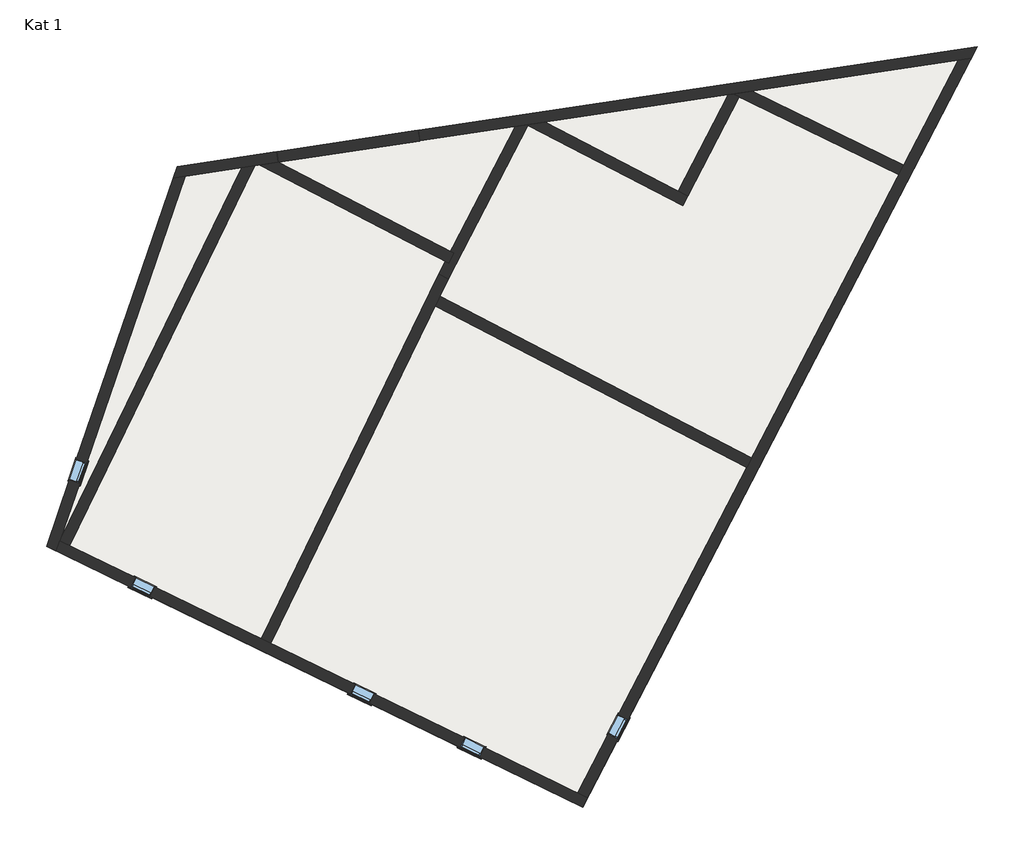
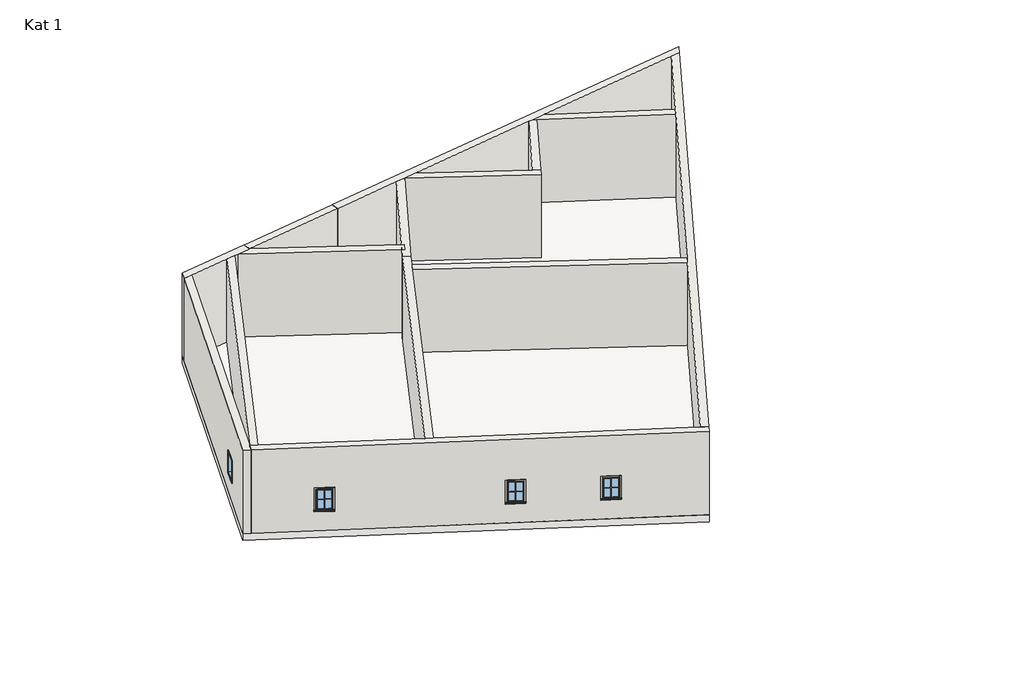
# One storey: 15 proxies, 14 walls, 5 windows, 1 slab.
"""IFC4 building model written with IfcOpenShell, lengths in millimetres."""

import ifcopenshell
import ifcopenshell.guid

model = None  # the IFC model being written
_history = None  # IfcOwnerHistory: only IFC2X3 demands one
_inside = {}  # id of a spatial element -> (the spatial element, [elements in it])
_under = {}  # id of a project, library or spatial element -> (it, [spatial elements below it])
_declared = {}  # id of a project -> (the project, [libraries it declares])
_typed = {}  # id of a type object -> (the type object, [elements of that type])
_made_of = {}  # id of a material, layer set ... -> (it, [elements and type objects made of it])


def new_model(schema):
    """Start an empty IFC model of exactly this schema.

    Asked for "IFC4X3", IfcOpenShell would pick the latest addendum, in which some entities
    have other attributes; the version numbers below select the first issue.
    IFC2X3 requires an IfcOwnerHistory on every rooted entity: one is made here for all.
    """
    global model, _history
    if schema == "IFC4X3":
        model = ifcopenshell.file(schema_version=(4, 3, 0, 0))
    else:
        model = ifcopenshell.file(schema=schema)
    _inside.clear()
    _under.clear()
    _declared.clear()
    _typed.clear()
    _made_of.clear()
    _history = None
    if model.schema == "IFC2X3":
        org = make("IfcOrganization", Name="unknown")
        user = make(
            "IfcPersonAndOrganization",
            ThePerson=make("IfcPerson", FamilyName="unknown"),
            TheOrganization=org,
        )
        app = make(
            "IfcApplication",
            ApplicationDeveloper=org,
            Version="unknown",
            ApplicationFullName="unknown",
            ApplicationIdentifier="unknown",
        )
        _history = make(
            "IfcOwnerHistory",
            OwningUser=user,
            OwningApplication=app,
            ChangeAction="ADDED",
            CreationDate=0,
        )
    return model


def make(cls, **values):
    """One entity of the class cls with the attributes given. An attribute that is None is left unset."""
    return model.create_entity(
        cls, **{name: value for name, value in values.items() if value is not None}
    )


def rooted(cls, **values):
    """An entity with a GlobalId (a new one), such as an element, a storey or a relation."""
    return make(cls, GlobalId=ifcopenshell.guid.new(), OwnerHistory=_history, **values)


def si_unit(unit_type, name, prefix=None):
    """IfcSIUnit, for example si_unit("LENGTHUNIT", "METRE", prefix="MILLI")."""
    return make("IfcSIUnit", UnitType=unit_type, Prefix=prefix, Name=name)


def assignment(units):
    """IfcUnitAssignment: the units of a project."""
    return None if units is None else make("IfcUnitAssignment", Units=units)


def point(xyz):
    """IfcCartesianPoint."""
    return None if xyz is None else make("IfcCartesianPoint", Coordinates=xyz)


def direction(xyz):
    """IfcDirection."""
    return None if xyz is None else make("IfcDirection", DirectionRatios=xyz)


def frame(location, z_axis=None, x_axis=None):
    """IfcAxis2Placement3D, a coordinate frame: its origin and axes. An axis left out is left unset."""
    return make(
        "IfcAxis2Placement3D",
        Location=point(location),
        Axis=direction(z_axis),
        RefDirection=direction(x_axis),
    )


def origin():
    """The frame at (0, 0, 0) with its axes left unset."""
    return frame((0.0, 0.0, 0.0))


def origin_with_axes():
    """The frame at (0, 0, 0) with the z axis (0, 0, 1) and the x axis (1, 0, 0) written out."""
    return frame((0.0, 0.0, 0.0), z_axis=(0.0, 0.0, 1.0), x_axis=(1.0, 0.0, 0.0))


def place(relative_to, where):
    """IfcLocalPlacement: puts the frame where relative to a parent placement (None: the world)."""
    return make(
        "IfcLocalPlacement", PlacementRelTo=relative_to, RelativePlacement=where
    )


def context(
    kind, dimensions, precision=None, world=None, true_north=None, identifier=None
):
    """IfcGeometricRepresentationContext, for example the 3D "Model" context."""
    return make(
        "IfcGeometricRepresentationContext",
        ContextIdentifier=identifier,
        ContextType=kind,
        CoordinateSpaceDimension=dimensions,
        Precision=precision,
        WorldCoordinateSystem=world,
        TrueNorth=true_north,
    )


def project(units=None, contexts=None):
    """IfcProject with its units and contexts."""
    return rooted(
        "IfcProject",
        Name="project",
        RepresentationContexts=contexts,
        UnitsInContext=assignment(units),
    )


def spatial(cls, under=None, at=None, **own):
    """A site, building, storey or space (cls), placed at a placement, below another one or the project."""
    s = rooted(cls, ObjectPlacement=at, **own)
    if under is not None:
        _under.setdefault(under.id(), (under, []))[1].append(s)
    return s


def polyline(points):
    """IfcPolyline through the points."""
    return make("IfcPolyline", Points=[point(p) for p in points])


def outline(outer, holes=None, kind="AREA"):
    """IfcArbitraryClosedProfileDef: a profile drawn as a closed curve; with holes, ...WithVoids."""
    if holes is None:
        return make("IfcArbitraryClosedProfileDef", ProfileType=kind, OuterCurve=outer)
    return make(
        "IfcArbitraryProfileDefWithVoids",
        ProfileType=kind,
        OuterCurve=outer,
        InnerCurves=holes,
    )


def extrude(swept, where, along, depth):
    """IfcExtrudedAreaSolid: the profile swept, set in the frame where, extruded along a direction by depth."""
    return make(
        "IfcExtrudedAreaSolid",
        SweptArea=swept,
        Position=where,
        ExtrudedDirection=direction(along),
        Depth=depth,
    )


def faces_of(points, faces, orient=None, outer=None):
    """IfcFace entities. A face is a list of loops; a loop is a list of indices into points, from 0.

    orient and outer hold one flag for each loop. By default every Orientation is true, the
    first loop of a face is its IfcFaceOuterBound and the others are IfcFaceBound.
    """
    made = []
    for i, loops in enumerate(faces):
        bounds = []
        for j, loop in enumerate(loops):
            is_outer = j == 0 if outer is None else outer[i][j]
            bounds.append(
                make(
                    "IfcFaceOuterBound" if is_outer else "IfcFaceBound",
                    Bound=make("IfcPolyLoop", Polygon=[points[k] for k in loop]),
                    Orientation=True if orient is None else orient[i][j],
                )
            )
        made.append(make("IfcFace", Bounds=bounds))
    return made


def faceted_brep(points, faces, orient=None, outer=None, voids=None):
    """IfcFacetedBrep: a solid bounded by flat faces; with voids (closed shells), ...WithVoids."""
    shared = [point(p) for p in points]
    hull = make("IfcClosedShell", CfsFaces=faces_of(shared, faces, orient, outer))
    if voids is None:
        return make("IfcFacetedBrep", Outer=hull)
    return make(
        "IfcFacetedBrepWithVoids",
        Outer=hull,
        Voids=[
            make(cls, CfsFaces=faces_of(shared, fs, o, b)) for cls, fs, o, b in voids
        ],
    )


def shape(context_of_items, identifier, shape_type, items):
    """IfcShapeRepresentation: the items that make up one representation, for example the "Body"."""
    return make(
        "IfcShapeRepresentation",
        ContextOfItems=context_of_items,
        RepresentationIdentifier=identifier,
        RepresentationType=shape_type,
        Items=items,
    )


def source(mapping_origin, context_of_items, identifier, shape_type, items):
    """IfcRepresentationMap: a shape defined once, which mapped items show again and again."""
    return make(
        "IfcRepresentationMap",
        MappingOrigin=mapping_origin,
        MappedRepresentation=shape(context_of_items, identifier, shape_type, items),
    )


def transform(
    local_origin,
    x_axis=None,
    y_axis=None,
    z_axis=None,
    scale=None,
    scale2=None,
    scale3=None,
    uniform=True,
):
    """IfcCartesianTransformationOperator3D, or its non-uniform kind. x_axis, y_axis, z_axis: its Axis1, 2, 3."""
    if uniform:
        return make(
            "IfcCartesianTransformationOperator3D",
            Axis1=direction(x_axis),
            Axis2=direction(y_axis),
            LocalOrigin=point(local_origin),
            Scale=scale,
            Axis3=direction(z_axis),
        )
    return make(
        "IfcCartesianTransformationOperator3DnonUniform",
        Axis1=direction(x_axis),
        Axis2=direction(y_axis),
        LocalOrigin=point(local_origin),
        Scale=scale,
        Axis3=direction(z_axis),
        Scale2=scale2,
        Scale3=scale3,
    )


def mapped(mapping_source, mapping_target):
    """IfcMappedItem: shows the shape of a source again, moved by a transform."""
    return make(
        "IfcMappedItem", MappingSource=mapping_source, MappingTarget=mapping_target
    )


def made_of(thing, what):
    """Note that an element or type object is made of a material, layer set ...; save() writes the relation."""
    if what is not None:
        _made_of.setdefault(what.id(), (what, []))[1].append(thing)
    return thing


def element(
    cls,
    number,
    at=None,
    inside=None,
    cuts=None,
    type_object=None,
    material=None,
    context=None,
    identifier="Body",
    shape_type=None,
    held_by="IfcProductDefinitionShape",
    body=None,
    shapes=None,
    **own,
):
    """One element of the class cls, such as IfcWall. Its Tag is "e" and its number.

    at: its placement. inside: the storey or other place that contains it. cuts: it is an
    opening in that element (IfcRelVoidsElement). A single representation is given by context,
    identifier, shape_type and body (its items); several are given by shapes. held_by: the class
    of the entity that holds the representations. save() writes the other relations.
    """
    e = rooted(cls, Tag="e%d" % number, ObjectPlacement=at, **own)
    if body is not None:
        shapes = [shape(context, identifier, shape_type, body)]
    if shapes is not None:
        e.Representation = make(held_by, Representations=shapes)
    if inside is not None:
        _inside.setdefault(inside.id(), (inside, []))[1].append(e)
    if cuts is not None:
        rooted(
            "IfcRelVoidsElement", RelatingBuildingElement=cuts, RelatedOpeningElement=e
        )
    if type_object is not None:
        _typed.setdefault(type_object.id(), (type_object, []))[1].append(e)
    return made_of(e, material)


def aggregate(whole, parts):
    """IfcRelAggregates: a whole, such as a stair, and the parts it consists of."""
    return rooted("IfcRelAggregates", RelatingObject=whole, RelatedObjects=parts)


def save(model, path):
    """Write the relations noted so far, then the file.

    IfcRelAggregates (storeys below a building ...), IfcRelContainedInSpatialStructure (elements
    in a storey), IfcRelDefinesByType, IfcRelAssociatesMaterial and IfcRelDeclares: one each for
    every whole, place, type object, material and project.
    """
    for whole, parts in _under.values():
        aggregate(whole, parts)
    for where, things in _inside.values():
        rooted(
            "IfcRelContainedInSpatialStructure",
            RelatedElements=things,
            RelatingStructure=where,
        )
    for kind, things in _typed.values():
        rooted("IfcRelDefinesByType", RelatedObjects=things, RelatingType=kind)
    for what, things in _made_of.values():
        rooted("IfcRelAssociatesMaterial", RelatedObjects=things, RelatingMaterial=what)
    for by, libraries in _declared.values():
        rooted("IfcRelDeclares", RelatingContext=by, RelatedDefinitions=libraries)
    model.write(path)


def m_muntin_pattern_2x2_m_muntin_pattern_2x2_8a7fc2d2(model_context):
    return source(origin(), model_context, "Body", "SweptSolid", [
        extrude(outline(polyline([(418.25, -6.35), (418.25, -261.9), (405.55, -261.9), (405.55, -6.35), (0.0, -6.35), (0.0, 6.35), (405.55, 6.35), (405.55, 261.9), (418.25, 261.9), (418.25, 6.35), (823.8, 6.35), (823.8, -6.35), (418.25, -6.35)])), frame((0.0, -22.225, 0.0), z_axis=(0.0, 1.0, 0.0), x_axis=(0.0, 0.0, 1.0)), (0.0, 0.0, 1.0), 12.7),
        extrude(outline(polyline([(418.25, -6.35), (418.25, -261.9), (405.55, -261.9), (405.55, -6.35), (0.0, -6.35), (0.0, 6.35), (405.55, 6.35), (405.55, 261.9), (418.25, 261.9), (418.25, 6.35), (823.8, 6.35), (823.8, -6.35), (418.25, -6.35)])), frame((0.0, 9.525, 0.0), z_axis=(0.0, 1.0, 0.0), x_axis=(0.0, 0.0, 1.0)), (0.0, 0.0, 1.0), 12.7),
    ])


def m_trim_window_exterior_flat_with_sill_a9fd4a74(model_context):
    return source(origin(), model_context, "Body", "SweptSolid", [
        extrude(outline(polyline([(360.0, -920.4323709), (360.0, -980.4323709), (-360.0, -980.4323709), (-360.0, -920.4323709), (360.0, -920.4323709)])), origin_with_axes(), (0.0, 0.0, 1.0), 19.05),
        extrude(outline(polyline([(-930.0, 38.1), (-902.4580645, 38.1), (-900.0, 19.05), (-900.0, 0.0), (-920.4323709, 0.0), (-920.4323709, 19.05), (-930.0, 19.05), (-930.0, 38.1)])), frame((-372.7, 0.0, 0.0), z_axis=(1.0, 0.0, 0.0), x_axis=(0.0, 1.0, 0.0)), (0.0, 0.0, 1.0), 745.4),
        extrude(outline(polyline([(-360.0, 60.0), (360.0, 60.0), (360.0, -900.0), (300.0, -900.0), (300.0, 0.0), (-300.0, 0.0), (-300.0, -900.0), (-360.0, -900.0), (-360.0, 60.0)])), origin_with_axes(), (0.0, 0.0, 1.0), 19.05),
    ])


def m_trim_window_interior_flat_picture_frame_0a41e60c(model_context):
    return source(origin(), model_context, "Body", "SweptSolid", [
        extrude(outline(polyline([(347.3, 47.3), (347.3, -947.3), (-347.3, -947.3), (-347.3, 47.3), (347.3, 47.3)]), holes=[polyline([(287.3, -12.7), (-287.3, -12.7), (-287.3, -887.3), (287.3, -887.3), (287.3, -12.7)])]), origin_with_axes(), (0.0, 0.0, 1.0), 30.0),
    ])


def m_window_fixed_600_x_900mm_140d34e2(model_context):
    return source(origin(), model_context, "Body", "SolidModel", [
        faceted_brep([(300.0, 54.75, 1800.0), (300.0, 169.05, 1800.0), (-300.0, 169.05, 1800.0), (-300.0, 54.75, 1800.0), (-300.0, 169.05, 900.0), (-300.0, 54.75, 900.0), (300.0, 169.05, 900.0), (300.0, 54.75, 900.0), (268.25, 54.75, 1768.25), (268.25, 54.75, 931.75), (-268.25, 54.75, 931.75), (-268.25, 54.75, 1768.25), (-287.3, 169.05, 1787.3), (-287.3, 169.05, 912.7), (287.3, 169.05, 912.7), (287.3, 169.05, 1787.3), (268.25, 118.25, 1768.25), (-268.25, 118.25, 1768.25), (287.3, 118.25, 1787.3), (-287.3, 118.25, 1787.3), (-268.25, 118.25, 931.75), (-287.3, 118.25, 912.7), (268.25, 118.25, 931.75), (287.3, 118.25, 912.7)], [[[0, 1, 2, 3]], [[3, 2, 4, 5]], [[5, 4, 6, 7]], [[3, 5, 7, 0], [8, 9, 10, 11]], [[7, 6, 1, 0]], [[1, 6, 4, 2], [12, 13, 14, 15]], [[16, 8, 11, 17]], [[15, 18, 19, 12]], [[17, 11, 10, 20]], [[12, 19, 21, 13]], [[20, 10, 9, 22]], [[13, 21, 23, 14]], [[22, 9, 8, 16]], [[18, 23, 21, 19], [17, 20, 22, 16]], [[14, 23, 18, 15]]]),
        extrude(outline(polyline([(1800.0, -300.0), (900.0, -300.0), (900.0, 300.0), (1800.0, 300.0), (1800.0, -300.0)]), holes=[polyline([(1787.3, 287.3), (912.7, 287.3), (912.7, -287.3), (1787.3, -287.3), (1787.3, 287.3)])]), frame((0.0, -150.0, 0.0), z_axis=(0.0, 1.0, 0.0), x_axis=(0.0, 0.0, 1.0)), (0.0, 0.0, 1.0), 204.75),
        extrude(outline(polyline([(912.7, 287.3), (1787.3, 287.3), (1787.3, -287.3), (912.7, -287.3), (912.7, 287.3)]), holes=[polyline([(938.1, -261.9), (1761.9, -261.9), (1761.9, 261.9), (938.1, 261.9), (938.1, -261.9)])]), frame((0.0, 118.25, 0.0), z_axis=(0.0, 1.0, 0.0), x_axis=(0.0, 0.0, 1.0)), (0.0, 0.0, 1.0), 44.45),
        extrude(outline(polyline([(261.9, 150.0), (261.9, 143.65), (-261.9, 143.65), (-261.9, 150.0), (261.9, 150.0)])), frame((0.0, 0.0, 938.1), z_axis=(0.0, 0.0, 1.0), x_axis=(1.0, 0.0, 0.0)), (0.0, 0.0, 1.0), 823.8),
        extrude(outline(polyline([(-261.9, 130.95), (-261.9, 137.3), (261.9, 137.3), (261.9, 130.95), (-261.9, 130.95)])), frame((0.0, 0.0, 938.1), z_axis=(0.0, 0.0, 1.0), x_axis=(1.0, 0.0, 0.0)), (0.0, 0.0, 1.0), 823.8),
    ])


model = new_model("IFC4")

# Units and contexts
model_context = context("Model", 3, world=origin())
ifc_project = project(units=[si_unit("LENGTHUNIT", "METRE", prefix="MILLI")], contexts=[model_context])

# Site, building, storey
site = spatial("IfcSite", under=ifc_project)
building = spatial("IfcBuilding", under=site)
storey = spatial("IfcBuildingStorey", under=building, Name="Kat 1", Elevation=15600.0)

# Proxies
placement = place(None, origin())
m_muntin_pattern_2x2_m_muntin_pattern_2x2_shape = m_muntin_pattern_2x2_m_muntin_pattern_2x2_8a7fc2d2(model_context)
element("IfcBuildingElementProxy", 1, Name="M_Muntin Pattern_2x2 : M_Muntin Pattern_2x2", ObjectType="M_Muntin Pattern_2x2 : M_Muntin Pattern_2x2", at=placement, inside=storey, context=model_context, shape_type="MappedRepresentation", body=[
    mapped(m_muntin_pattern_2x2_m_muntin_pattern_2x2_shape, transform((102257.299698, 48021.0608967, 16538.1), x_axis=(0.8990027605086794, -0.43794296043865577, 0.0), y_axis=(0.43794296043865577, 0.8990027605086794, 0.0), z_axis=(0.0, 0.0, 1.0))),
])
element("IfcBuildingElementProxy", 2, Name="M_Muntin Pattern_2x2 : M_Muntin Pattern_2x2", ObjectType="M_Muntin Pattern_2x2 : M_Muntin Pattern_2x2", at=placement, inside=storey, context=model_context, shape_type="MappedRepresentation", body=[
    mapped(m_muntin_pattern_2x2_m_muntin_pattern_2x2_shape, transform((108370.5184694, 45043.0487657, 16538.1), x_axis=(0.8990027605086794, -0.43794296043865577, 0.0), y_axis=(0.43794296043865577, 0.8990027605086794, 0.0), z_axis=(0.0, 0.0, 1.0))),
])
element("IfcBuildingElementProxy", 3, Name="M_Muntin Pattern_2x2 : M_Muntin Pattern_2x2", ObjectType="M_Muntin Pattern_2x2 : M_Muntin Pattern_2x2", at=placement, inside=storey, context=model_context, shape_type="MappedRepresentation", body=[
    mapped(m_muntin_pattern_2x2_m_muntin_pattern_2x2_shape, transform((111427.1278552, 43554.0427002, 16538.1), x_axis=(0.8990027605086794, -0.43794296043865577, 0.0), y_axis=(0.43794296043865577, 0.8990027605086794, 0.0), z_axis=(0.0, 0.0, 1.0))),
])
element("IfcBuildingElementProxy", 4, Name="M_Muntin Pattern_2x2 : M_Muntin Pattern_2x2", ObjectType="M_Muntin Pattern_2x2 : M_Muntin Pattern_2x2", at=placement, inside=storey, context=model_context, shape_type="MappedRepresentation", body=[
    mapped(m_muntin_pattern_2x2_m_muntin_pattern_2x2_shape, transform((115678.8068066, 44189.9755294, 16538.1), x_axis=(0.46062188620761896, 0.8875964612066315, 0.0), y_axis=(-0.8875964612066315, 0.46062188620761896, 0.0), z_axis=(0.0, 0.0, 1.0))),
])
element("IfcBuildingElementProxy", 5, Name="M_Muntin Pattern_2x2 : M_Muntin Pattern_2x2", ObjectType="M_Muntin Pattern_2x2 : M_Muntin Pattern_2x2", at=placement, inside=storey, context=model_context, shape_type="MappedRepresentation", body=[
    mapped(m_muntin_pattern_2x2_m_muntin_pattern_2x2_shape, transform((100646.9467086, 51326.3991966, 16538.1), x_axis=(0.3253074083155791, 0.9456083174840423, 0.0), y_axis=(-0.9456083174840423, 0.3253074083155791, 0.0), z_axis=(0.0, 0.0, 1.0))),
])
m_trim_window_exterior_flat_with_sill_shape = m_trim_window_exterior_flat_with_sill_a9fd4a74(model_context)
element("IfcBuildingElementProxy", 6, Name="M_Trim-Window-Exterior-Flat : with Sill", ObjectType="M_Trim-Window-Exterior-Flat : with Sill", at=placement, inside=storey, context=model_context, shape_type="MappedRepresentation", body=[
    mapped(m_trim_window_exterior_flat_with_sill_shape, transform((102253.1282913, 48012.4978954, 17400.0), x_axis=(0.8990027605086794, -0.43794296043865577, 0.0), y_axis=(0.0, 0.0, 1.0), z_axis=(-0.43794296043865577, -0.8990027605086794, 0.0))),
])
element("IfcBuildingElementProxy", 7, Name="M_Trim-Window-Exterior-Flat : with Sill", ObjectType="M_Trim-Window-Exterior-Flat : with Sill", at=placement, inside=storey, context=model_context, shape_type="MappedRepresentation", body=[
    mapped(m_trim_window_exterior_flat_with_sill_shape, transform((108366.3470627, 45034.4857644, 17400.0), x_axis=(0.8990027605086794, -0.43794296043865577, 0.0), y_axis=(0.0, 0.0, 1.0), z_axis=(-0.43794296043865577, -0.8990027605086794, 0.0))),
])
element("IfcBuildingElementProxy", 8, Name="M_Trim-Window-Exterior-Flat : with Sill", ObjectType="M_Trim-Window-Exterior-Flat : with Sill", at=placement, inside=storey, context=model_context, shape_type="MappedRepresentation", body=[
    mapped(m_trim_window_exterior_flat_with_sill_shape, transform((111422.9564485, 43545.4796989, 17400.0), x_axis=(0.8990027605086794, -0.43794296043865577, 0.0), y_axis=(0.0, 0.0, 1.0), z_axis=(-0.43794296043865577, -0.8990027605086794, 0.0))),
])
element("IfcBuildingElementProxy", 9, Name="M_Trim-Window-Exterior-Flat : with Sill", ObjectType="M_Trim-Window-Exterior-Flat : with Sill", at=placement, inside=storey, context=model_context, shape_type="MappedRepresentation", body=[
    mapped(m_trim_window_exterior_flat_with_sill_shape, transform((115687.2611629, 44185.5881059, 17400.0), x_axis=(0.46062188620761896, 0.8875964612066315, 0.0), y_axis=(0.0, 0.0, 1.0), z_axis=(0.8875964612066315, -0.46062188620761896, 0.0))),
])
element("IfcBuildingElementProxy", 10, Name="M_Trim-Window-Exterior-Flat : with Sill", ObjectType="M_Trim-Window-Exterior-Flat : with Sill", at=placement, inside=storey, context=model_context, shape_type="MappedRepresentation", body=[
    mapped(m_trim_window_exterior_flat_with_sill_shape, transform((100655.9536279, 51323.3006435, 17400.0), x_axis=(0.3253074083155791, 0.9456083174840423, 0.0), y_axis=(0.0, 0.0, 1.0), z_axis=(0.9456083174840423, -0.3253074083155791, 0.0))),
])
m_trim_window_interior_flat_picture_frame_shape = m_trim_window_interior_flat_picture_frame_0a41e60c(model_context)
element("IfcBuildingElementProxy", 11, Name="M_Trim-Window-Interior-Flat : Picture Frame", ObjectType="M_Trim-Window-Interior-Flat : Picture Frame", at=placement, inside=storey, context=model_context, shape_type="MappedRepresentation", body=[
    mapped(m_trim_window_interior_flat_picture_frame_shape, transform((102384.5111794, 48282.1987235, 17400.0), x_axis=(-0.8990027605086794, 0.43794296043865577, 0.0), y_axis=(0.0, 0.0, 1.0), z_axis=(0.43794296043865577, 0.8990027605086794, 0.0))),
])
element("IfcBuildingElementProxy", 12, Name="M_Trim-Window-Interior-Flat : Picture Frame", ObjectType="M_Trim-Window-Interior-Flat : Picture Frame", at=placement, inside=storey, context=model_context, shape_type="MappedRepresentation", body=[
    mapped(m_trim_window_interior_flat_picture_frame_shape, transform((108497.7299509, 45304.1865926, 17400.0), x_axis=(-0.8990027605086794, 0.43794296043865577, 0.0), y_axis=(0.0, 0.0, 1.0), z_axis=(0.43794296043865577, 0.8990027605086794, 0.0))),
])
element("IfcBuildingElementProxy", 13, Name="M_Trim-Window-Interior-Flat : Picture Frame", ObjectType="M_Trim-Window-Interior-Flat : Picture Frame", at=placement, inside=storey, context=model_context, shape_type="MappedRepresentation", body=[
    mapped(m_trim_window_interior_flat_picture_frame_shape, transform((111554.3393366, 43815.1805271, 17400.0), x_axis=(-0.8990027605086794, 0.43794296043865577, 0.0), y_axis=(0.0, 0.0, 1.0), z_axis=(0.43794296043865577, 0.8990027605086794, 0.0))),
])
element("IfcBuildingElementProxy", 14, Name="M_Trim-Window-Interior-Flat : Picture Frame", ObjectType="M_Trim-Window-Interior-Flat : Picture Frame", at=placement, inside=storey, context=model_context, shape_type="MappedRepresentation", body=[
    mapped(m_trim_window_interior_flat_picture_frame_shape, transform((115420.9822245, 44323.7746718, 17400.0), x_axis=(-0.46062188620761896, -0.8875964612066315, 0.0), y_axis=(0.0, 0.0, 1.0), z_axis=(-0.8875964612066315, 0.46062188620761896, 0.0))),
])
element("IfcBuildingElementProxy", 15, Name="M_Trim-Window-Interior-Flat : Picture Frame", ObjectType="M_Trim-Window-Interior-Flat : Picture Frame", at=placement, inside=storey, context=model_context, shape_type="MappedRepresentation", body=[
    mapped(m_trim_window_interior_flat_picture_frame_shape, transform((100372.2711326, 51420.892866, 17400.0), x_axis=(-0.3253074083155791, -0.9456083174840423, 0.0), y_axis=(0.0, 0.0, 1.0), z_axis=(-0.9456083174840423, 0.3253074083155791, 0.0))),
])

# Slab
element("IfcSlab", 16, ObjectType="Generic - 12\"", at=placement, inside=storey, context=model_context, shape_type="SweptSolid", body=[
    extrude(outline(polyline([(103277.4815183, 59865.8007732), (125559.0390197, 63208.0343984), (114561.6077302, 42016.5074927), (99637.9813419, 49286.4485964), (103277.4815183, 59865.8007732)])), frame((0.0, 0.0, 15295.2), z_axis=(0.0, 0.0, 1.0), x_axis=(1.0, 0.0, 0.0)), (0.0, 0.0, 1.0), 304.8),
])

# Walls
element("IfcWall", 17, ObjectType="Generic - 300mm Masonry", at=placement, inside=storey, context=model_context, shape_type="Brep", body=[
    faceted_brep([(103167.4428423, 59545.9387455, 15600.0), (103501.9610368, 59596.1164747, 15600.0), (105070.1496085, 59831.3447604, 15600.0), (105430.15912, 59885.3461872, 15600.0), (105581.2339042, 59908.0074048, 15600.0), (106078.6437378, 59982.6188798, 15600.0), (106078.6437378, 59982.6188798, 19200.0), (105581.2339042, 59908.0074048, 19200.0), (105430.15912, 59885.3461872, 19200.0), (105070.1496085, 59831.3447604, 19200.0), (103501.9610368, 59596.1164747, 19200.0), (103167.4428423, 59545.9387455, 19200.0), (103277.4815183, 59865.8007732, 15600.0), (103277.4815183, 59865.8007732, 19200.0), (106034.1416019, 60279.2997857, 19200.0), (106034.1416019, 60279.2997857, 15600.0)], [[[0, 1, 2, 3, 4, 5, 6, 7, 8, 9, 10, 11]], [[12, 13, 14, 15]], [[5, 4, 3, 2, 1, 0, 12, 15]], [[6, 5, 15, 14]], [[11, 10, 9, 8, 7, 6, 14, 13]], [[0, 11, 13, 12]]]),
])
element("IfcWall", 18, ObjectType="Generic - 300mm Masonry", at=placement, inside=storey, context=model_context, shape_type="Brep", body=[
    faceted_brep([(99909.7008895, 49154.0823031, 15600.0), (100008.0235929, 49439.888171, 15600.0), (103501.9610368, 59596.1164747, 15600.0), (103501.9610368, 59596.1164747, 19200.0), (100008.0235929, 49439.888171, 19200.0), (99909.7008895, 49154.0823031, 19200.0), (100558.3614054, 51039.6181483, 17400.0), (100753.5458504, 51606.9831388, 17400.0), (100753.5458504, 51606.9831388, 16500.0), (100558.3614054, 51039.6181483, 16500.0), (99637.9813419, 49286.4485964, 15600.0), (99637.9813419, 49286.4485964, 19200.0), (103167.4428423, 59545.9387455, 19200.0), (103167.4428423, 59545.9387455, 15600.0), (100274.6789101, 51137.2103708, 17400.0), (100274.6789101, 51137.2103708, 16500.0), (100469.8633551, 51704.5753613, 16500.0), (100469.8633551, 51704.5753613, 17400.0)], [[[0, 1, 2, 3, 4, 5], [6, 7, 8, 9]], [[10, 11, 12, 13], [14, 15, 16, 17]], [[2, 1, 0, 10, 13]], [[5, 4, 3, 12, 11]], [[3, 2, 13, 12]], [[0, 5, 11, 10]], [[15, 14, 6, 9]], [[16, 15, 9, 8]], [[17, 16, 8, 7]], [[14, 17, 7, 6]]]),
])
element("IfcWall", 19, ObjectType="Generic - 300mm Masonry", at=placement, inside=storey, context=model_context, shape_type="Brep", body=[
    faceted_brep([(114699.8388367, 42282.8722588, 15600.0), (114430.0510779, 42414.2974946, 15600.0), (105879.9744511, 46579.4080308, 15600.0), (105610.273623, 46710.790919, 15600.0), (100277.724421, 49308.5052829, 15600.0), (100008.0235929, 49439.888171, 15600.0), (100008.0235929, 49439.888171, 19200.0), (100277.724421, 49308.5052829, 19200.0), (105610.273623, 46710.790919, 19200.0), (105879.9744511, 46579.4080308, 19200.0), (114430.0510779, 42414.2974946, 19200.0), (114699.8388367, 42282.8722588, 19200.0), (102114.8103513, 48413.5816117, 17400.0), (102114.8103513, 48413.5816117, 16500.0), (102654.2120076, 48150.8158354, 16500.0), (102654.2120076, 48150.8158354, 17400.0), (108228.0291227, 45435.5694807, 17400.0), (108228.0291227, 45435.5694807, 16500.0), (108767.430779, 45172.8037044, 16500.0), (108767.430779, 45172.8037044, 17400.0), (111284.6385084, 43946.5634152, 17400.0), (111284.6385084, 43946.5634152, 16500.0), (111824.0401648, 43683.7976389, 16500.0), (111824.0401648, 43683.7976389, 17400.0), (114561.6077302, 42016.5074927, 15600.0), (114561.6077302, 42016.5074927, 19200.0), (99909.7008895, 49154.0823031, 19200.0), (99909.7008895, 49154.0823031, 15600.0), (101983.4274631, 48143.8807835, 17400.0), (102522.8291194, 47881.1150073, 17400.0), (102522.8291194, 47881.1150073, 16500.0), (101983.4274631, 48143.8807835, 16500.0), (108096.6462346, 45165.8686525, 17400.0), (108636.0478909, 44903.1028763, 17400.0), (108636.0478909, 44903.1028763, 16500.0), (108096.6462346, 45165.8686525, 16500.0), (111153.2556203, 43676.862587, 17400.0), (111692.6572766, 43414.0968108, 17400.0), (111692.6572766, 43414.0968108, 16500.0), (111153.2556203, 43676.862587, 16500.0)], [[[0, 1, 2, 3, 4, 5, 6, 7, 8, 9, 10, 11], [12, 13, 14, 15], [16, 17, 18, 19], [20, 21, 22, 23]], [[24, 25, 26, 27], [28, 29, 30, 31], [32, 33, 34, 35], [36, 37, 38, 39]], [[5, 4, 3, 2, 1, 0, 24, 27]], [[11, 10, 9, 8, 7, 6, 26, 25]], [[6, 5, 27, 26]], [[0, 11, 25, 24]], [[13, 12, 28, 31]], [[14, 13, 31, 30]], [[15, 14, 30, 29]], [[12, 15, 29, 28]], [[17, 16, 32, 35]], [[18, 17, 35, 34]], [[19, 18, 34, 33]], [[16, 19, 33, 32]], [[21, 20, 36, 39]], [[22, 21, 39, 38]], [[23, 22, 38, 37]], [[20, 23, 37, 36]]]),
])
element("IfcWall", 20, ObjectType="Generic - 300mm Masonry", at=placement, inside=storey, context=model_context, shape_type="Brep", body=[
    faceted_brep([(125021.7991789, 62824.092196, 15600.0), (123507.1408189, 59905.4175942, 15600.0), (123368.9097124, 59639.0528281, 15600.0), (119271.3649828, 51743.2790697, 15600.0), (119133.1784169, 51477.0001314, 15600.0), (114430.0510779, 42414.2974946, 15600.0), (114430.0510779, 42414.2974946, 19200.0), (119133.1784169, 51477.0001314, 19200.0), (119271.3649828, 51743.2790697, 19200.0), (123368.9097124, 59639.0528281, 19200.0), (123507.1408189, 59905.4175942, 19200.0), (125021.7991789, 62824.092196, 19200.0), (115282.7956586, 44057.4957334, 17400.0), (115282.7956586, 44057.4957334, 16500.0), (115559.1687904, 44590.0536101, 16500.0), (115559.1687904, 44590.0536101, 17400.0), (125388.3218852, 62879.070602, 15600.0), (125388.3218852, 62879.070602, 19200.0), (114699.8388367, 42282.8722588, 19200.0), (114699.8388367, 42282.8722588, 15600.0), (115549.074597, 43919.3091675, 17400.0), (115825.4477287, 44451.8670443, 17400.0), (115825.4477287, 44451.8670443, 16500.0), (115549.074597, 43919.3091675, 16500.0)], [[[0, 1, 2, 3, 4, 5, 6, 7, 8, 9, 10, 11], [12, 13, 14, 15]], [[16, 17, 18, 19], [20, 21, 22, 23]], [[5, 4, 3, 2, 1, 0, 16, 19]], [[11, 10, 9, 8, 7, 6, 18, 17]], [[6, 5, 19, 18]], [[13, 12, 20, 23]], [[14, 13, 23, 22]], [[15, 14, 22, 21]], [[12, 15, 21, 20]], [[0, 11, 17, 16]]]),
])
element("IfcWall", 21, ObjectType="Generic - 300mm Masonry", at=placement, inside=storey, context=model_context, shape_type="Brep", body=[
    faceted_brep([(123507.1408189, 59905.4175942, 15600.0), (119282.8527515, 61963.2502319, 15600.0), (119282.8527515, 61963.2502319, 19200.0), (123507.1408189, 59905.4175942, 19200.0), (123368.9097124, 59639.0528281, 15600.0), (123368.9097124, 59639.0528281, 19200.0), (118924.0603327, 61804.3303796, 19200.0), (118759.1036766, 61884.6878707, 19200.0), (118759.1036766, 61884.6878707, 15600.0), (118924.0603327, 61804.3303796, 15600.0)], [[[0, 1, 2, 3]], [[4, 5, 6, 7, 8, 9]], [[1, 0, 4, 9, 8]], [[3, 2, 7, 6, 5]], [[2, 1, 8, 7]], [[0, 3, 5, 4]]]),
])
element("IfcWall", 22, ObjectType="Generic - 300mm Masonry", at=placement, inside=storey, context=model_context, shape_type="SweptSolid", body=[
    extrude(outline(polyline([(117223.7741184, 59179.2531459), (118616.6843925, 61863.324978), (118759.1036766, 61884.6878707), (118924.0603327, 61804.3303796), (117490.0530567, 59041.06658), (117223.7741184, 59179.2531459)])), frame((0.0, 0.0, 15600.0), z_axis=(0.0, 0.0, 1.0), x_axis=(1.0, 0.0, 0.0)), (0.0, 0.0, 1.0), 3600.0),
])
element("IfcWall", 23, ObjectType="Generic - 300mm Masonry", at=placement, inside=storey, context=model_context, shape_type="Brep", body=[
    faceted_brep([(113045.6890264, 61009.4964003, 15600.0), (117351.8664909, 58774.7876417, 15600.0), (117351.8664909, 58774.7876417, 19200.0), (113045.6890264, 61009.4964003, 19200.0), (113523.7668589, 61099.387348, 15600.0), (113523.7668589, 61099.387348, 19200.0), (117223.7741184, 59179.2531459, 19200.0), (117490.0530567, 59041.06658, 19200.0), (117490.0530567, 59041.06658, 15600.0), (117223.7741184, 59179.2531459, 15600.0), (113055.919617, 61029.2102617, 15600.0), (113055.919617, 61029.2102617, 19200.0)], [[[0, 1, 2, 3]], [[4, 5, 6, 7, 8, 9]], [[1, 0, 10, 4, 9, 8]], [[3, 2, 7, 6, 5, 11]], [[0, 3, 11, 10]], [[11, 5, 4, 10]], [[2, 1, 8, 7]]]),
])
element("IfcWall", 24, ObjectType="Generic - 300mm Masonry", at=placement, inside=storey, context=model_context, shape_type="Brep", body=[
    faceted_brep([(105581.2339042, 59908.0074048, 15600.0), (110837.5728904, 57180.2083607, 15600.0), (110837.5728904, 57180.2083607, 19200.0), (105581.2339042, 59908.0074048, 19200.0), (106086.4873992, 59983.7954291, 15600.0), (106086.4873992, 59983.7954291, 19200.0), (110975.7594563, 57446.4872991, 19200.0), (110975.7594563, 57446.4872991, 15600.0), (106078.6437378, 59982.6188798, 15600.0), (106078.6437378, 59982.6188798, 19200.0)], [[[0, 1, 2, 3]], [[4, 5, 6, 7]], [[1, 0, 8, 4, 7]], [[2, 1, 7, 6]], [[3, 2, 6, 5, 9]], [[0, 3, 9, 5, 4, 8]]]),
])
element("IfcWall", 25, ObjectType="Generic - 300mm Masonry", at=placement, inside=storey, context=model_context, shape_type="Brep", body=[
    faceted_brep([(110823.8219249, 56728.0641982, 15600.0), (113045.6890264, 61009.4964003, 15600.0), (113055.919617, 61029.2102617, 15600.0), (113055.919617, 61029.2102617, 19200.0), (113045.6890264, 61009.4964003, 19200.0), (110823.8219249, 56728.0641982, 19200.0), (110555.788859, 56862.8706438, 15600.0), (110555.788859, 56862.8706438, 19200.0), (112689.3969107, 60974.2318558, 19200.0), (112689.3969107, 60974.2318558, 15600.0)], [[[0, 1, 2, 3, 4, 5]], [[6, 7, 8, 9]], [[2, 1, 0, 6, 9]], [[5, 4, 3, 8, 7]], [[3, 2, 9, 8]], [[0, 5, 7, 6]]]),
])
element("IfcWall", 26, ObjectType="Generic - 300mm Masonry", at=placement, inside=storey, context=model_context, shape_type="Brep", body=[
    faceted_brep([(110555.788859, 56862.8706438, 15600.0), (105610.273623, 46710.790919, 15600.0), (105610.273623, 46710.790919, 19200.0), (110555.788859, 56862.8706438, 19200.0), (110823.8219249, 56728.0641982, 15600.0), (110823.8219249, 56728.0641982, 19200.0), (110590.1678223, 56248.4225503, 19200.0), (110458.7425865, 55978.6347915, 19200.0), (105879.9744511, 46579.4080308, 19200.0), (105879.9744511, 46579.4080308, 15600.0), (110458.7425865, 55978.6347915, 15600.0), (110590.1678223, 56248.4225503, 15600.0)], [[[0, 1, 2, 3]], [[4, 5, 6, 7, 8, 9, 10, 11]], [[1, 0, 4, 11, 10, 9]], [[3, 2, 8, 7, 6, 5]], [[2, 1, 9, 8]], [[0, 3, 5, 4]]]),
])
element("IfcWall", 27, ObjectType="Generic - 300mm Masonry", at=placement, inside=storey, context=model_context, shape_type="SweptSolid", body=[
    extrude(outline(polyline([(105430.15912, 59885.3461872), (100277.724421, 49308.5052829), (100008.0235929, 49439.888171), (105070.1496085, 59831.3447604), (105430.15912, 59885.3461872)])), frame((0.0, 0.0, 15600.0), z_axis=(0.0, 0.0, 1.0), x_axis=(1.0, 0.0, 0.0)), (0.0, 0.0, 1.0), 3600.0),
])
element("IfcWall", 28, ObjectType="Generic - 300mm Masonry", at=placement, inside=storey, context=model_context, shape_type="SweptSolid", body=[
    extrude(outline(polyline([(119133.1784169, 51477.0001314), (110458.7425865, 55978.6347915), (110590.1678223, 56248.4225503), (119271.3649828, 51743.2790697), (119133.1784169, 51477.0001314)])), frame((0.0, 0.0, 15600.0), z_axis=(0.0, 0.0, 1.0), x_axis=(1.0, 0.0, 0.0)), (0.0, 0.0, 1.0), 3600.0),
])
element("IfcWall", 29, ObjectType="Generic - 300mm Masonry", at=placement, inside=storey, context=model_context, shape_type="SweptSolid", body=[
    extrude(outline(polyline([(110024.9464958, 60574.5642935), (106103.3671466, 59986.3273912), (106058.8650107, 60283.008297), (109980.4443599, 60871.2451994), (110024.9464958, 60574.5642935)])), frame((0.0, 0.0, 15600.0), z_axis=(0.0, 0.0, 1.0), x_axis=(1.0, 0.0, 0.0)), (0.0, 0.0, 1.0), 3600.0),
])
element("IfcWall", 30, ObjectType="Generic - 300mm Masonry", at=placement, inside=storey, context=model_context, shape_type="Brep", body=[
    faceted_brep([(110049.6699046, 60578.2728049, 15600.0), (112689.3969107, 60974.2318558, 15600.0), (113055.919617, 61029.2102617, 15600.0), (113523.7668589, 61099.387348, 15600.0), (118616.6843925, 61863.324978, 15600.0), (118759.1036766, 61884.6878707, 15600.0), (119282.8527515, 61963.2502319, 15600.0), (125021.7991789, 62824.092196, 15600.0), (125388.3218852, 62879.070602, 15600.0), (125388.3218852, 62879.070602, 19200.0), (125021.7991789, 62824.092196, 19200.0), (119282.8527515, 61963.2502319, 19200.0), (118759.1036766, 61884.6878707, 19200.0), (118616.6843925, 61863.324978, 19200.0), (113523.7668589, 61099.387348, 19200.0), (113055.919617, 61029.2102617, 19200.0), (112689.3969107, 60974.2318558, 19200.0), (110049.6699046, 60578.2728049, 19200.0), (110005.1677687, 60874.9537107, 15600.0), (110005.1677687, 60874.9537107, 19200.0), (125559.0390197, 63208.0343984, 19200.0), (125559.0390197, 63208.0343984, 15600.0)], [[[0, 1, 2, 3, 4, 5, 6, 7, 8, 9, 10, 11, 12, 13, 14, 15, 16, 17]], [[18, 19, 20, 21]], [[8, 7, 6, 5, 4, 3, 2, 1, 0, 18, 21]], [[17, 16, 15, 14, 13, 12, 11, 10, 9, 20, 19]], [[0, 17, 19, 18]], [[9, 8, 21, 20]]]),
])

# Windows
m_window_fixed_600_x_900mm_shape = m_window_fixed_600_x_900mm_140d34e2(model_context)
element("IfcWindow", 31, ObjectType="M_Window-Fixed : 600 x 900mm", at=placement, inside=storey, context=model_context, shape_type="MappedRepresentation", body=[
    mapped(m_window_fixed_600_x_900mm_shape, transform((102318.8197353, 48147.3483095, 15600.0), x_axis=(-0.8990027605086794, 0.43794296043865577, 0.0), y_axis=(-0.43794296043865577, -0.8990027605086794, 0.0), z_axis=(0.0, 0.0, 1.0))),
])
element("IfcWindow", 32, ObjectType="M_Window-Fixed : 600 x 900mm", at=placement, inside=storey, context=model_context, shape_type="MappedRepresentation", body=[
    mapped(m_window_fixed_600_x_900mm_shape, transform((108432.0385068, 45169.3361785, 15600.0), x_axis=(-0.8990027605086794, 0.43794296043865577, 0.0), y_axis=(-0.43794296043865577, -0.8990027605086794, 0.0), z_axis=(0.0, 0.0, 1.0))),
])
element("IfcWindow", 33, ObjectType="M_Window-Fixed : 600 x 900mm", at=placement, inside=storey, context=model_context, shape_type="MappedRepresentation", body=[
    mapped(m_window_fixed_600_x_900mm_shape, transform((111488.6478925, 43680.330113, 15600.0), x_axis=(-0.8990027605086794, 0.43794296043865577, 0.0), y_axis=(-0.43794296043865577, -0.8990027605086794, 0.0), z_axis=(0.0, 0.0, 1.0))),
])
element("IfcWindow", 34, ObjectType="M_Window-Fixed : 600 x 900mm", at=placement, inside=storey, context=model_context, shape_type="MappedRepresentation", body=[
    mapped(m_window_fixed_600_x_900mm_shape, transform((115554.1216937, 44254.6813888, 15600.0), x_axis=(-0.46062188620761896, -0.8875964612066315, 0.0), y_axis=(0.8875964612066315, -0.46062188620761896, 0.0), z_axis=(0.0, 0.0, 1.0))),
])
element("IfcWindow", 35, ObjectType="M_Window-Fixed : 600 x 900mm", at=placement, inside=storey, context=model_context, shape_type="MappedRepresentation", body=[
    mapped(m_window_fixed_600_x_900mm_shape, transform((100514.1123802, 51372.0967548, 15600.0), x_axis=(-0.3253074083155791, -0.9456083174840423, 0.0), y_axis=(0.9456083174840423, -0.3253074083155791, 0.0), z_axis=(0.0, 0.0, 1.0))),
])

save(model, "model.ifc")

# Revit data of these elements
# Type "M_Muntin Pattern_2x2 : M_Muntin Pattern_2x2"
#   Width [instance default] = 120 cm
#   Thickness = 1.27 cm
#   Height [instance default] = 120 cm
#   Distance = 1.905 cm
#   Interior Material [instance default] = none
#   Exterior Material [instance default] = none
#   Default Elevation = 0
# Type "M_Trim-Window-Exterior-Flat : with Sill"
#   Trim Width = 6 cm
#   Trim Thickness_Picture Frame = 3 cm
#   Trim Thickness_with Sill = 1.905 cm
#   Sill Thickness = 3 cm
#   Opening Width [instance default] = 60 cm
#   Opening Height [instance default] = 90 cm
#   Default Elevation = 120 cm
#   Sill = yes
#   Picture Frame = no
#   Trim Material [instance default] = none
# Type "M_Trim-Window-Interior-Flat : Picture Frame"
#   Trim Thickness_Picture Frame = 3 cm
#   Trim Width = 6 cm
#   Trim Thickness_with Sill = 2 cm
#   Sill Thickness = 3 cm
#   Opening Width [instance default] = 60 cm
#   Opening Height [instance default] = 90 cm
#   Default Elevation = 120 cm
#   Sill = no
#   Picture Frame = yes
#   Trim Material [instance default] = none
# Type "Generic - 12\""
#   Description = "Generic Floor (Material By Category), 12\" thick"
#   Assembly Code = "B1010"
#   Type Mark = "G01"
#   Function = 0
#   Layers, outside or top first: 30.48 cm no material (function 1)
# Type "Generic - 300mm Masonry"
#   Description = "Generic Wall (Material By Category), 300mm thick, Masonry pattern"
#   Assembly Code = "B2010"
#   Type Mark = "G10"
#   Layers, outside or top first: 30 cm "Gravel" (function 1)
# Type "M_Window-Fixed : 600 x 900mm"
#   Type Mark = "32"
#   Fire Rating = "0.5h"
#   Assembly Code = "B2020100"
#   Analytic Construction = "Double glazing - domestic"
#   Window Inset [instance default] = 0 cm
#   Wall Thickness [instance default] = 15 cm
#   Visual Light Transmittance = 0.81
#   Thermal Resistance (R) = 0.319569 (m²·K)/W
#   Solar Heat Gain Coefficient = 0.76
#   Rough Width = 61.5 cm
#   Rough Height = 91.5 cm
#   Interior Wall Closure [instance default] = 5.475 cm
#   Height = 90 cm
#   Heat Transfer Coefficient (U) = 3.12929 W/(m²·K)
#   Frame Extension [instance default] = 0.635 cm
#   Exterior Wall Closure [instance default] = 3.175 cm
#   Extension Jamb [instance default] = 5.475 cm
#   Default Sill Height = 90 cm
#   Width = 60 cm
#   Muntin Visibility = yes
#   Interior Trim Visibility [instance default] = yes
#   Exterior Trim Visibility [instance default] = yes
#   Extension Jamb Visibility [instance default] = yes
#   Muntin Pattern = M_Muntin Pattern_2x2 : M_Muntin Pattern_2x2
#   Interior Trim Material = Wood - Stained
#   Interior Trim = M_Trim-Window-Interior-Flat : Picture Frame
#   Interior Frame Material = Wood - Stained
#   Glass Panel Material = Glass
#   Exterior Trim Material = Clad - White
#   Exterior Trim = M_Trim-Window-Exterior-Flat : with Sill
#   Exterior Frame Material = Clad - White
#   Wall Closure = (empty or 0)
# Elements 1, 2, 3, 4, 5 (IfcBuildingElementProxy, "M_Muntin Pattern_2x2 : M_Muntin Pattern_2x2")
#   Width = 52.38 cm
#   Height = 82.38 cm
#   Interior Material = Wood - Stained
#   Exterior Material = Clad - White
#   Phase Created = New Construction
#   Materials on its faces: "Clad - White", "Wood - Stained"
# Elements 6, 7, 8, 9, 10 (IfcBuildingElementProxy, "M_Trim-Window-Exterior-Flat : with Sill")
#   Opening Width = 60 cm
#   Opening Height = 90 cm
#   Trim Material = Clad - White
#   Phase Created = New Construction
#   Materials on its faces: "Clad - White"
# Elements 11, 12, 13, 14, 15 (IfcBuildingElementProxy, "M_Trim-Window-Interior-Flat : Picture Frame")
#   Opening Width = 60 cm
#   Opening Height = 90 cm
#   Trim Material = Wood - Stained
#   Phase Created = New Construction
#   Materials on its faces: "Wood - Stained"
# Element 16 (IfcSlab, "Generic - 12\"")
#   built-in parameter 1001955 = -2.9927 (stored number, unit not read)
#   Height Offset From Level = 0 cm
#   Phase Created = New Construction
#   Materials on its faces: "Default Floor"
# Elements 17, 18, 19, 20, 21, 22, 23, 24, 25, 26, 27, 28, 29, 30 (IfcWall, "Generic - 300mm Masonry")
#   Top Offset = 0 cm
#   Base Offset = 0 cm
#   wall height = 360 cm
#   Phase Created = New Construction
#   Base Constraint = Kat 1
#   Top Constraint = Kat 2
#   Materials on its faces: "Gravel"
# Element 31 (IfcWindow, "M_Window-Fixed : 600 x 900mm")
#   Mark = "100"
#   Window Inset = 0 cm
#   Interior Wall Closure = 5.475 cm
#   Frame Extension = 0.635 cm
#   Exterior Wall Closure = 3.175 cm
#   Interior Trim Visibility = yes
#   Exterior Trim Visibility = yes
#   Phase Created = New Construction
#   Materials on its faces: "Wood - Stained", "Glass", "Clad - White"
# Element 32 (IfcWindow, "M_Window-Fixed : 600 x 900mm")
#   Mark = "102"
#   Window Inset = 0 cm
#   Interior Wall Closure = 5.475 cm
#   Frame Extension = 0.635 cm
#   Exterior Wall Closure = 3.175 cm
#   Interior Trim Visibility = yes
#   Exterior Trim Visibility = yes
#   Phase Created = New Construction
#   Materials on its faces: "Wood - Stained", "Glass", "Clad - White"
# Element 33 (IfcWindow, "M_Window-Fixed : 600 x 900mm")
#   Mark = "103"
#   Window Inset = 0 cm
#   Interior Wall Closure = 5.475 cm
#   Frame Extension = 0.635 cm
#   Exterior Wall Closure = 3.175 cm
#   Interior Trim Visibility = yes
#   Exterior Trim Visibility = yes
#   Phase Created = New Construction
#   Materials on its faces: "Wood - Stained", "Glass", "Clad - White"
# Element 34 (IfcWindow, "M_Window-Fixed : 600 x 900mm")
#   Mark = "104"
#   Window Inset = 0 cm
#   Interior Wall Closure = 5.475 cm
#   Frame Extension = 0.635 cm
#   Exterior Wall Closure = 3.175 cm
#   Interior Trim Visibility = yes
#   Exterior Trim Visibility = yes
#   Phase Created = New Construction
#   Materials on its faces: "Wood - Stained", "Glass", "Clad - White"
# Element 35 (IfcWindow, "M_Window-Fixed : 600 x 900mm")
#   Mark = "105"
#   Window Inset = 0 cm
#   Interior Wall Closure = 5.475 cm
#   Frame Extension = 0.635 cm
#   Exterior Wall Closure = 3.175 cm
#   Interior Trim Visibility = yes
#   Exterior Trim Visibility = yes
#   Phase Created = New Construction
#   Materials on its faces: "Wood - Stained", "Glass", "Clad - White"
# Materials
#   "Gravel": class "Generic", colour RGB 120 120 120, transparency 0, Description = "Crushed stone or gravel", Cost = 0
#   "Wood - Stained": class "Wood", colour RGB 173 132 96, transparency 0, Cost = 0
#   "Glass": class "Glass", colour RGB 245 245 243, transparency 1, Description = "Soda Lime Glass", Cost = 0
#   "Clad - White": class "Wood", colour RGB 245 245 243, transparency 0, Cost = 0
#   "Default Floor": class "Miscellaneous", colour RGB 128 128 128, transparency 0, Cost = 0
# Room, not placed, phase "New Construction", upper offset 0 cm, lower offset 0 cm
#   Number = "103"
#   Name = "Room Name"
# Room at (105123.467, 54653.445) mm, phase "New Construction", upper level "Kat 1", upper offset 304.8 cm, lower offset 0 cm
#   Number = ""
#   Name = "Room Name"
# Room at (118831.075, 57352.874) mm, phase "New Construction", upper level "Kat 1", upper offset 304.8 cm, lower offset 0 cm
#   Number = ""
#   Name = "Room Name"
# Room, not placed, phase "New Construction", upper offset 0 cm, lower offset 0 cm
#   Number = ""
#   Name = "Room Name"
# Room, not placed, phase "New Construction", upper offset 0 cm, lower offset 0 cm
#   Number = "."
#   Name = "Room Name"
# Room, not placed, phase "New Construction", upper offset 0 cm, lower offset 0 cm
#   Number = "108"
#   Name = "Room Name"
# Room at (112024.655, 51089.261) mm, phase "New Construction", upper level "Kat 1", upper offset 304.8 cm, lower offset 0 cm
#   Number = "109"
#   Name = "Room Name"
# Room at (103957.349, 59237.211) mm, phase "New Construction", upper level "Kat 1", upper offset 304.8 cm, lower offset 0 cm
#   Number = ""
#   Name = "Room Name"
# Room at (122677.349, 61812.956) mm, phase "New Construction", upper level "Kat 1", upper offset 304.8 cm, lower offset 0 cm
#   Number = ""
#   Name = "Room Name"
# Room at (116622.696, 61380.481) mm, phase "New Construction", upper level "Kat 1", upper offset 304.8 cm, lower offset 0 cm
#   Number = ""
#   Name = "Room Name"
# Room at (109768.655, 59692.271) mm, phase "New Construction", upper level "Kat 1", upper offset 304.8 cm, lower offset 0 cm
#   Number = ""
#   Name = "Room Name"
